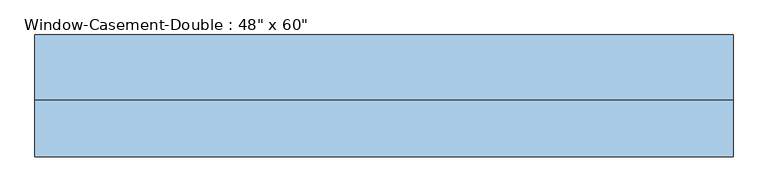
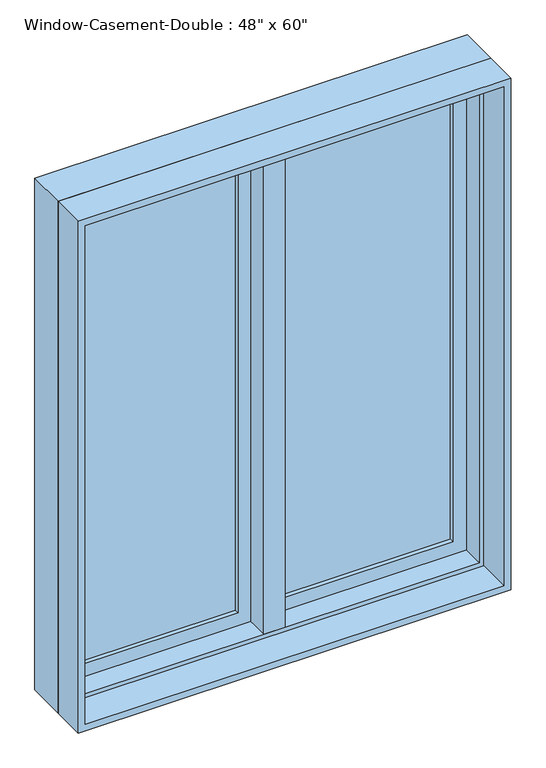
"""IFC4 building model written with IfcOpenShell, lengths in millimetres: window geometry."""

import ifcopenshell
import ifcopenshell.guid

model = None  # the IFC model being written
_history = None  # IfcOwnerHistory: only IFC2X3 demands one
_inside = {}  # id of a spatial element -> (the spatial element, [elements in it])
_under = {}  # id of a project, library or spatial element -> (it, [spatial elements below it])
_declared = {}  # id of a project -> (the project, [libraries it declares])
_typed = {}  # id of a type object -> (the type object, [elements of that type])
_made_of = {}  # id of a material, layer set ... -> (it, [elements and type objects made of it])


def new_model(schema):
    """Start an empty IFC model of exactly this schema.

    Asked for "IFC4X3", IfcOpenShell would pick the latest addendum, in which some entities
    have other attributes; the version numbers below select the first issue.
    IFC2X3 requires an IfcOwnerHistory on every rooted entity: one is made here for all.
    """
    global model, _history
    if schema == "IFC4X3":
        model = ifcopenshell.file(schema_version=(4, 3, 0, 0))
    else:
        model = ifcopenshell.file(schema=schema)
    _inside.clear()
    _under.clear()
    _declared.clear()
    _typed.clear()
    _made_of.clear()
    _history = None
    if model.schema == "IFC2X3":
        org = make("IfcOrganization", Name="unknown")
        user = make(
            "IfcPersonAndOrganization",
            ThePerson=make("IfcPerson", FamilyName="unknown"),
            TheOrganization=org,
        )
        app = make(
            "IfcApplication",
            ApplicationDeveloper=org,
            Version="unknown",
            ApplicationFullName="unknown",
            ApplicationIdentifier="unknown",
        )
        _history = make(
            "IfcOwnerHistory",
            OwningUser=user,
            OwningApplication=app,
            ChangeAction="ADDED",
            CreationDate=0,
        )
    return model


def make(cls, **values):
    """One entity of the class cls with the attributes given. An attribute that is None is left unset."""
    return model.create_entity(
        cls, **{name: value for name, value in values.items() if value is not None}
    )


def rooted(cls, **values):
    """An entity with a GlobalId (a new one), such as an element, a storey or a relation."""
    return make(cls, GlobalId=ifcopenshell.guid.new(), OwnerHistory=_history, **values)


def si_unit(unit_type, name, prefix=None):
    """IfcSIUnit, for example si_unit("LENGTHUNIT", "METRE", prefix="MILLI")."""
    return make("IfcSIUnit", UnitType=unit_type, Prefix=prefix, Name=name)


def assignment(units):
    """IfcUnitAssignment: the units of a project."""
    return None if units is None else make("IfcUnitAssignment", Units=units)


def point(xyz):
    """IfcCartesianPoint."""
    return None if xyz is None else make("IfcCartesianPoint", Coordinates=xyz)


def direction(xyz):
    """IfcDirection."""
    return None if xyz is None else make("IfcDirection", DirectionRatios=xyz)


def frame(location, z_axis=None, x_axis=None):
    """IfcAxis2Placement3D, a coordinate frame: its origin and axes. An axis left out is left unset."""
    return make(
        "IfcAxis2Placement3D",
        Location=point(location),
        Axis=direction(z_axis),
        RefDirection=direction(x_axis),
    )


def origin():
    """The frame at (0, 0, 0) with its axes left unset."""
    return frame((0.0, 0.0, 0.0))


def place(relative_to, where):
    """IfcLocalPlacement: puts the frame where relative to a parent placement (None: the world)."""
    return make(
        "IfcLocalPlacement", PlacementRelTo=relative_to, RelativePlacement=where
    )


def context(
    kind, dimensions, precision=None, world=None, true_north=None, identifier=None
):
    """IfcGeometricRepresentationContext, for example the 3D "Model" context."""
    return make(
        "IfcGeometricRepresentationContext",
        ContextIdentifier=identifier,
        ContextType=kind,
        CoordinateSpaceDimension=dimensions,
        Precision=precision,
        WorldCoordinateSystem=world,
        TrueNorth=true_north,
    )


def project(units=None, contexts=None):
    """IfcProject with its units and contexts."""
    return rooted(
        "IfcProject",
        Name="project",
        RepresentationContexts=contexts,
        UnitsInContext=assignment(units),
    )


def spatial(cls, under=None, at=None, **own):
    """A site, building, storey or space (cls), placed at a placement, below another one or the project."""
    s = rooted(cls, ObjectPlacement=at, **own)
    if under is not None:
        _under.setdefault(under.id(), (under, []))[1].append(s)
    return s


def polyline(points):
    """IfcPolyline through the points."""
    return make("IfcPolyline", Points=[point(p) for p in points])


def outline(outer, holes=None, kind="AREA"):
    """IfcArbitraryClosedProfileDef: a profile drawn as a closed curve; with holes, ...WithVoids."""
    if holes is None:
        return make("IfcArbitraryClosedProfileDef", ProfileType=kind, OuterCurve=outer)
    return make(
        "IfcArbitraryProfileDefWithVoids",
        ProfileType=kind,
        OuterCurve=outer,
        InnerCurves=holes,
    )


def extrude(swept, where, along, depth):
    """IfcExtrudedAreaSolid: the profile swept, set in the frame where, extruded along a direction by depth."""
    return make(
        "IfcExtrudedAreaSolid",
        SweptArea=swept,
        Position=where,
        ExtrudedDirection=direction(along),
        Depth=depth,
    )


def faces_of(points, faces, orient=None, outer=None):
    """IfcFace entities. A face is a list of loops; a loop is a list of indices into points, from 0.

    orient and outer hold one flag for each loop. By default every Orientation is true, the
    first loop of a face is its IfcFaceOuterBound and the others are IfcFaceBound.
    """
    made = []
    for i, loops in enumerate(faces):
        bounds = []
        for j, loop in enumerate(loops):
            is_outer = j == 0 if outer is None else outer[i][j]
            bounds.append(
                make(
                    "IfcFaceOuterBound" if is_outer else "IfcFaceBound",
                    Bound=make("IfcPolyLoop", Polygon=[points[k] for k in loop]),
                    Orientation=True if orient is None else orient[i][j],
                )
            )
        made.append(make("IfcFace", Bounds=bounds))
    return made


def faceted_brep(points, faces, orient=None, outer=None, voids=None):
    """IfcFacetedBrep: a solid bounded by flat faces; with voids (closed shells), ...WithVoids."""
    shared = [point(p) for p in points]
    hull = make("IfcClosedShell", CfsFaces=faces_of(shared, faces, orient, outer))
    if voids is None:
        return make("IfcFacetedBrep", Outer=hull)
    return make(
        "IfcFacetedBrepWithVoids",
        Outer=hull,
        Voids=[
            make(cls, CfsFaces=faces_of(shared, fs, o, b)) for cls, fs, o, b in voids
        ],
    )


def shape(context_of_items, identifier, shape_type, items):
    """IfcShapeRepresentation: the items that make up one representation, for example the "Body"."""
    return make(
        "IfcShapeRepresentation",
        ContextOfItems=context_of_items,
        RepresentationIdentifier=identifier,
        RepresentationType=shape_type,
        Items=items,
    )


def source(mapping_origin, context_of_items, identifier, shape_type, items):
    """IfcRepresentationMap: a shape defined once, which mapped items show again and again."""
    return make(
        "IfcRepresentationMap",
        MappingOrigin=mapping_origin,
        MappedRepresentation=shape(context_of_items, identifier, shape_type, items),
    )


def transform(
    local_origin,
    x_axis=None,
    y_axis=None,
    z_axis=None,
    scale=None,
    scale2=None,
    scale3=None,
    uniform=True,
):
    """IfcCartesianTransformationOperator3D, or its non-uniform kind. x_axis, y_axis, z_axis: its Axis1, 2, 3."""
    if uniform:
        return make(
            "IfcCartesianTransformationOperator3D",
            Axis1=direction(x_axis),
            Axis2=direction(y_axis),
            LocalOrigin=point(local_origin),
            Scale=scale,
            Axis3=direction(z_axis),
        )
    return make(
        "IfcCartesianTransformationOperator3DnonUniform",
        Axis1=direction(x_axis),
        Axis2=direction(y_axis),
        LocalOrigin=point(local_origin),
        Scale=scale,
        Axis3=direction(z_axis),
        Scale2=scale2,
        Scale3=scale3,
    )


def mapped(mapping_source, mapping_target):
    """IfcMappedItem: shows the shape of a source again, moved by a transform."""
    return make(
        "IfcMappedItem", MappingSource=mapping_source, MappingTarget=mapping_target
    )


def made_of(thing, what):
    """Note that an element or type object is made of a material, layer set ...; save() writes the relation."""
    if what is not None:
        _made_of.setdefault(what.id(), (what, []))[1].append(thing)
    return thing


def element(
    cls,
    number,
    at=None,
    inside=None,
    cuts=None,
    type_object=None,
    material=None,
    context=None,
    identifier="Body",
    shape_type=None,
    held_by="IfcProductDefinitionShape",
    body=None,
    shapes=None,
    **own,
):
    """One element of the class cls, such as IfcWall. Its Tag is "e" and its number.

    at: its placement. inside: the storey or other place that contains it. cuts: it is an
    opening in that element (IfcRelVoidsElement). A single representation is given by context,
    identifier, shape_type and body (its items); several are given by shapes. held_by: the class
    of the entity that holds the representations. save() writes the other relations.
    """
    e = rooted(cls, Tag="e%d" % number, ObjectPlacement=at, **own)
    if body is not None:
        shapes = [shape(context, identifier, shape_type, body)]
    if shapes is not None:
        e.Representation = make(held_by, Representations=shapes)
    if inside is not None:
        _inside.setdefault(inside.id(), (inside, []))[1].append(e)
    if cuts is not None:
        rooted(
            "IfcRelVoidsElement", RelatingBuildingElement=cuts, RelatedOpeningElement=e
        )
    if type_object is not None:
        _typed.setdefault(type_object.id(), (type_object, []))[1].append(e)
    return made_of(e, material)


def aggregate(whole, parts):
    """IfcRelAggregates: a whole, such as a stair, and the parts it consists of."""
    return rooted("IfcRelAggregates", RelatingObject=whole, RelatedObjects=parts)


def save(model, path):
    """Write the relations noted so far, then the file.

    IfcRelAggregates (storeys below a building ...), IfcRelContainedInSpatialStructure (elements
    in a storey), IfcRelDefinesByType, IfcRelAssociatesMaterial and IfcRelDeclares: one each for
    every whole, place, type object, material and project.
    """
    for whole, parts in _under.values():
        aggregate(whole, parts)
    for where, things in _inside.values():
        rooted(
            "IfcRelContainedInSpatialStructure",
            RelatedElements=things,
            RelatingStructure=where,
        )
    for kind, things in _typed.values():
        rooted("IfcRelDefinesByType", RelatedObjects=things, RelatingType=kind)
    for what, things in _made_of.values():
        rooted("IfcRelAssociatesMaterial", RelatedObjects=things, RelatingMaterial=what)
    for by, libraries in _declared.values():
        rooted("IfcRelDeclares", RelatingContext=by, RelatedDefinitions=libraries)
    model.write(path)


def window_d7f95d13(model_context):
    return source(origin(), model_context, "Body", "SolidModel", [
        faceted_brep([(9.525, 115.8875, 2425.7), (-9.525, 115.8875, 2425.7), (-9.525, 65.0875, 2425.7), (9.525, 65.0875, 2425.7), (9.525, 115.8875, 927.1), (9.525, 65.0875, 927.1), (-9.525, 65.0875, 927.1), (-9.525, 115.8875, 927.1), (-9.525, 65.0875, 946.15), (-9.525, 65.0875, 2406.65), (-30.1625, 65.0875, 946.15), (-30.1625, 65.0875, 2406.65), (-30.1625, 1.5875, 946.15), (-30.1625, 1.5875, 2406.65), (30.1625, 1.5875, 946.15), (30.1625, 1.5875, 2406.65), (30.1625, 65.0875, 946.15), (30.1625, 65.0875, 2406.65), (9.525, 65.0875, 946.15), (9.525, 65.0875, 2406.65)], [[[0, 1, 2, 3]], [[4, 5, 6, 7]], [[1, 0, 4, 7]], [[2, 1, 7, 6, 8, 9]], [[9, 8, 10, 11]], [[11, 10, 12, 13]], [[13, 12, 14, 15]], [[15, 14, 16, 17]], [[17, 16, 18, 19]], [[0, 3, 19, 18, 5, 4]], [[18, 8, 6, 5]], [[9, 19, 3, 2]], [[8, 18, 16, 14, 12, 10]], [[19, 9, 11, 13, 15, 17]]]),
        extrude(outline(polyline([(-66.675, 96.8375), (-66.675, 90.4875), (-539.75, 90.4875), (-539.75, 96.8375), (-66.675, 96.8375)])), frame((0.0, 0.0, 984.25), z_axis=(0.0, 0.0, 1.0), x_axis=(1.0, 0.0, 0.0)), (0.0, 0.0, 1.0), 1384.3),
        extrude(outline(polyline([(-539.75, 77.7875), (-539.75, 84.1375), (-66.675, 84.1375), (-66.675, 77.7875), (-539.75, 77.7875)])), frame((0.0, 0.0, 984.25), z_axis=(0.0, 0.0, 1.0), x_axis=(1.0, 0.0, 0.0)), (0.0, 0.0, 1.0), 1384.3),
        extrude(outline(polyline([(539.75, 96.8375), (539.75, 90.4875), (66.675, 90.4875), (66.675, 96.8375), (539.75, 96.8375)])), frame((0.0, 0.0, 984.25), z_axis=(0.0, 0.0, 1.0), x_axis=(1.0, 0.0, 0.0)), (0.0, 0.0, 1.0), 1384.3),
        extrude(outline(polyline([(66.675, 77.7875), (66.675, 84.1375), (539.75, 84.1375), (539.75, 77.7875), (66.675, 77.7875)])), frame((0.0, 0.0, 984.25), z_axis=(0.0, 0.0, 1.0), x_axis=(1.0, 0.0, 0.0)), (0.0, 0.0, 1.0), 1384.3),
        extrude(outline(polyline([(2425.7, -596.9), (927.1, -596.9), (927.1, -9.525), (2425.7, -9.525), (2425.7, -596.9)]), holes=[polyline([(2368.55, -66.675), (984.25, -66.675), (984.25, -539.75), (2368.55, -539.75), (2368.55, -66.675)])]), frame((0.0, 65.0875, 0.0), z_axis=(0.0, 1.0, 0.0), x_axis=(0.0, 0.0, 1.0)), (0.0, 0.0, 1.0), 44.45),
        extrude(outline(polyline([(927.1, 596.9), (2425.7, 596.9), (2425.7, 9.525), (927.1, 9.525), (927.1, 596.9)]), holes=[polyline([(984.25, 66.675), (2368.55, 66.675), (2368.55, 539.75), (984.25, 539.75), (984.25, 66.675)])]), frame((0.0, 65.0875, 0.0), z_axis=(0.0, 1.0, 0.0), x_axis=(0.0, 0.0, 1.0)), (0.0, 0.0, 1.0), 44.45),
        extrude(outline(polyline([(2438.4, -609.6), (914.4, -609.6), (914.4, 609.6), (2438.4, 609.6), (2438.4, -609.6)]), holes=[polyline([(2419.35, 590.55), (933.45, 590.55), (933.45, -590.55), (2419.35, -590.55), (2419.35, 590.55)])]), frame((0.0, -96.8375, 0.0), z_axis=(0.0, 1.0, 0.0), x_axis=(0.0, 0.0, 1.0)), (0.0, 0.0, 1.0), 98.425),
        faceted_brep([(577.85, 65.0875, 2406.65), (577.85, 1.5875, 2406.65), (-577.85, 1.5875, 2406.65), (-577.85, 65.0875, 2406.65), (596.9, 115.8875, 2425.7), (596.9, 65.0875, 2425.7), (-596.9, 65.0875, 2425.7), (-596.9, 115.8875, 2425.7), (609.6, 1.5875, 2438.4), (609.6, 115.8875, 2438.4), (-609.6, 115.8875, 2438.4), (-609.6, 1.5875, 2438.4), (-577.85, 1.5875, 946.15), (-577.85, 65.0875, 946.15), (-596.9, 65.0875, 927.1), (-596.9, 115.8875, 927.1), (-609.6, 115.8875, 914.4), (-609.6, 1.5875, 914.4), (577.85, 1.5875, 946.15), (577.85, 65.0875, 946.15), (596.9, 65.0875, 927.1), (596.9, 115.8875, 927.1), (609.6, 115.8875, 914.4), (609.6, 1.5875, 914.4)], [[[0, 1, 2, 3]], [[4, 5, 6, 7]], [[8, 9, 10, 11]], [[3, 2, 12, 13]], [[7, 6, 14, 15]], [[11, 10, 16, 17]], [[13, 12, 18, 19]], [[15, 14, 20, 21]], [[17, 16, 22, 23]], [[11, 17, 23, 8], [1, 18, 12, 2]], [[19, 18, 1, 0]], [[5, 20, 14, 6], [3, 13, 19, 0]], [[21, 20, 5, 4]], [[23, 22, 9, 8]], [[9, 22, 16, 10], [7, 15, 21, 4]]]),
    ])


if __name__ == "__main__":
    model = new_model("IFC4")
    model_context = context("Model", 3, world=origin())
    ifc_project = project(units=[si_unit("LENGTHUNIT", "METRE", prefix="MILLI")], contexts=[model_context])
    site = spatial("IfcSite", under=ifc_project)
    building = spatial("IfcBuilding", under=site)
    placement = place(None, origin())
    window_shape = window_d7f95d13(model_context)
    element("IfcWindow", 1, ObjectType="Window-Casement-Double : 48\" x 60\"", at=placement, inside=building, context=model_context, shape_type="MappedRepresentation", body=[
        mapped(window_shape, transform((0.0, 0.0, 0.0), x_axis=(1.0, 0.0, 0.0), y_axis=(0.0, 1.0, 0.0), z_axis=(0.0, 0.0, 1.0))),
    ])
    save(model, "model.ifc")

# Revit data of these elements
# Type "Window-Casement-Double : 48\" x 60\""
#   Type Mark = "61"
#   Fire Rating = "0.5h"
#   Assembly Code = "B2020100"
#   Analytic Construction = "Double glazing - domestic"
#   Frame Extension [instance default] = 0' - 0 1/4"
#   Window Inset [instance default] = 0' - 0"
#   Wall Thickness [instance default] = 0' - 6"
#   Interior Wall Closure [instance default] = 0' - 2 1/4"
#   Half Width = 2' - 0"
#   Visual Light Transmittance = 0.81
#   Thermal Resistance (R) = 1.8146 (h·ft²·°F)/BTU
#   Solar Heat Gain Coefficient = 0.76
#   Rough Width = 4' - 0 1/2"
#   Rough Height = 5' - 0 1/2"
#   Height = 5' - 0"
#   Heat Transfer Coefficient (U) = 0.5511 BTU/(h·ft²·°F)
#   Exterior Wall Closure [instance default] = 0' - 1 1/4"
#   Extension Jamb [instance default] = 0' - 2 1/4"
#   Default Sill Height = 3' - 0"
#   Width = 4' - 0"
#   Define Thermal Properties by = 0
#   Muntin Visibility = yes
#   Interior Trim Visibility [instance default] = yes
#   Exterior Trim Visibility [instance default] = yes
#   Extension Jamb Visibility [instance default] = yes
#   Interior Trim Material = Wood - Stained
#   Muntin Pattern = Muntin Pattern_2x2 : Muntin Pattern_2x2
#   Interior Trim = Trim-Window-Interior-Flat : Picture Frame
#   Interior Frame Material = Wood - Stained
#   Glass Panel Material = Glass
#   Exterior Trim Material = Clad - White
#   Exterior Trim = Trim-Window-Exterior-Flat : with Sill
#   Exterior Frame Material = Clad - White
#   Wall Closure = (empty or 0)
# Element 1 (IfcWindow, "Window-Casement-Double : 48\" x 60\"")
#   Wall Thickness = 0' - 7 5/8"
#   Extension Jamb = 0' - 3 7/8"
#   Materials on its faces: "Wood - Stained", "Glass", "Clad - White"
# Materials
#   "Wood - Stained": class "Wood", colour RGB 224 178 126, transparency 0, Cost = 0
#   "Glass": class "Glass", colour RGB 236 240 239, transparency 0.5, Description = "Soda Lime Glass", Cost = 0
#   "Clad - White": class "Wood", colour RGB 216 216 204, transparency 0, Cost = 0
